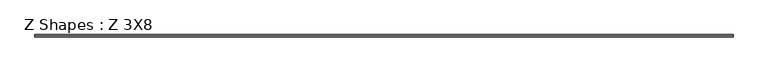
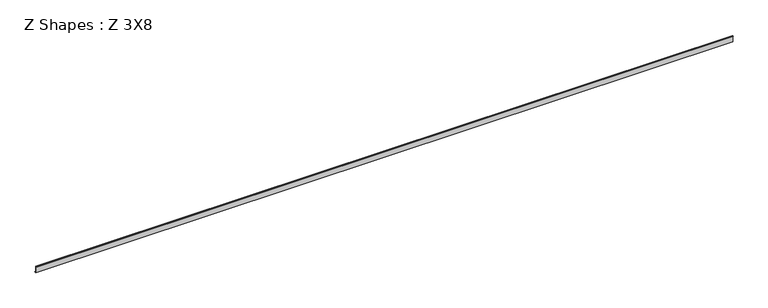
"""IFC4 building model written with IfcOpenShell, lengths in millimetres: beam geometry, Z Shapes : Z 3X8."""

from ifc_helpers import new_model, si_unit, frame, origin, place, context, project, spatial, polyline, outline, extrude, source, transform, mapped, element, save


def z_shapes_z_3x8_0ff4bf34(model_context):
    return source(origin(), model_context, "Body", "SweptSolid", [
        extrude(outline(polyline([(-57.2805719, 101.596825), (-57.2805719, 111.248825), (-19.1805719, 111.248825), (-19.1805719, -101.603175), (18.9194281, -101.603175), (18.9194281, -107.953175), (-27.1991352, -107.953175), (-27.1991352, 101.596825), (-57.2805719, 101.596825)])), frame((-11963.4, 0.0, 0.0), z_axis=(1.0, 0.0, 0.0), x_axis=(0.0, 1.0, 0.0)), (0.0, 0.0, 1.0), 23926.8),
    ])


if __name__ == "__main__":
    model = new_model("IFC4")
    model_context = context("Model", 3, world=origin())
    ifc_project = project(units=[si_unit("LENGTHUNIT", "METRE", prefix="MILLI")], contexts=[model_context])
    site = spatial("IfcSite", under=ifc_project)
    building = spatial("IfcBuilding", under=site)
    placement = place(None, origin())
    z_shapes_z_3x8_shape = z_shapes_z_3x8_0ff4bf34(model_context)
    element("IfcBeam", 1, ObjectType="Z Shapes : Z 3X8", at=placement, inside=building, context=model_context, shape_type="MappedRepresentation", body=[
        mapped(z_shapes_z_3x8_shape, transform((0.0, 0.0, 0.0), x_axis=(1.0, 0.0, 0.0), y_axis=(0.0, 1.0, 0.0), z_axis=(0.0, 0.0, 1.0))),
    ])
    save(model, "model.ifc")

# Revit data of these elements
# Type "Z Shapes : Z 3X8"
#   Section Name Key = "W12x26"
#   Assembly Code = "B10"
#   Width = 76.2 mm
#   Web Thickness = 5.842 mm
#   Web Fillet = 7.62 mm
#   Warping Constant = 163001.3 cm⁶
#   Torsional Moment of Inertia = 12.4869 cm⁴
#   Section Area = 7.65 in²
#   Plastic Modulus weak axis = 0.00472801 (stored number, unit not read)
#   Plastic Modulus strong axis = 0.0215278 (stored number, unit not read)
#   Perimeter = 15.0571 m²/m
#   Nominal Weight = 379.441 N/m
#   Moment of Inertia weak axis = 720.08 cm⁴
#   Moment of Inertia strong axis = 8491.12 cm⁴
#   Height = 203.2 mm
#   Flange Thickness = 9.652 mm
#   Elastic Modulus weak axis = 0.00309028 (stored number, unit not read)
#   Elastic Modulus strong axis = 0.0193287 (stored number, unit not read)
#   Centroid Vertical = 101.6 mm
#   Centroid Horizontal = 38.1 mm
#   Length [instance default] = 5' - 0"
#   Structural Material [instance default] = Steel ASTM A992
#   Principal Axes Angle = 0
# Element 1 (IfcBeam, "Z Shapes : Z 3X8")
#   Materials on its faces: "Steel ASTM A992"
# Materials
#   "Steel ASTM A992": class "Metal", colour RGB 189 187 185, transparency 0, Description = "Structural steel 50ksi", Cost = 0
